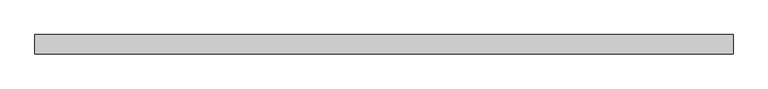
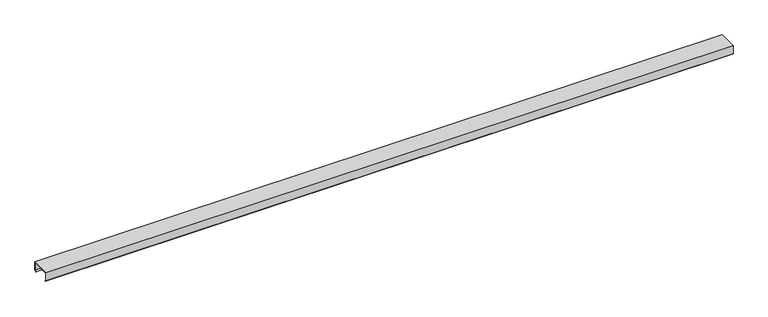
"""IFC4 building model written with IfcOpenShell, lengths in millimetres: proxy geometry, Generic Models 7:Generic Models 1:1:Generic Models 1:1 : Generic Models 7:Generic Models 1:337419:17 : Generic Models 7:Generic Models 1:1:Generic Models 1:1 : Generic Models 7:Generic Models 1:337419:306201."""

import ifcopenshell
import ifcopenshell.guid

model = None  # the IFC model being written
_history = None  # IfcOwnerHistory: only IFC2X3 demands one
_inside = {}  # id of a spatial element -> (the spatial element, [elements in it])
_under = {}  # id of a project, library or spatial element -> (it, [spatial elements below it])
_declared = {}  # id of a project -> (the project, [libraries it declares])
_typed = {}  # id of a type object -> (the type object, [elements of that type])
_made_of = {}  # id of a material, layer set ... -> (it, [elements and type objects made of it])


def new_model(schema):
    """Start an empty IFC model of exactly this schema.

    Asked for "IFC4X3", IfcOpenShell would pick the latest addendum, in which some entities
    have other attributes; the version numbers below select the first issue.
    IFC2X3 requires an IfcOwnerHistory on every rooted entity: one is made here for all.
    """
    global model, _history
    if schema == "IFC4X3":
        model = ifcopenshell.file(schema_version=(4, 3, 0, 0))
    else:
        model = ifcopenshell.file(schema=schema)
    _inside.clear()
    _under.clear()
    _declared.clear()
    _typed.clear()
    _made_of.clear()
    _history = None
    if model.schema == "IFC2X3":
        org = make("IfcOrganization", Name="unknown")
        user = make(
            "IfcPersonAndOrganization",
            ThePerson=make("IfcPerson", FamilyName="unknown"),
            TheOrganization=org,
        )
        app = make(
            "IfcApplication",
            ApplicationDeveloper=org,
            Version="unknown",
            ApplicationFullName="unknown",
            ApplicationIdentifier="unknown",
        )
        _history = make(
            "IfcOwnerHistory",
            OwningUser=user,
            OwningApplication=app,
            ChangeAction="ADDED",
            CreationDate=0,
        )
    return model


def make(cls, **values):
    """One entity of the class cls with the attributes given. An attribute that is None is left unset."""
    return model.create_entity(
        cls, **{name: value for name, value in values.items() if value is not None}
    )


def rooted(cls, **values):
    """An entity with a GlobalId (a new one), such as an element, a storey or a relation."""
    return make(cls, GlobalId=ifcopenshell.guid.new(), OwnerHistory=_history, **values)


def si_unit(unit_type, name, prefix=None):
    """IfcSIUnit, for example si_unit("LENGTHUNIT", "METRE", prefix="MILLI")."""
    return make("IfcSIUnit", UnitType=unit_type, Prefix=prefix, Name=name)


def assignment(units):
    """IfcUnitAssignment: the units of a project."""
    return None if units is None else make("IfcUnitAssignment", Units=units)


def point(xyz):
    """IfcCartesianPoint."""
    return None if xyz is None else make("IfcCartesianPoint", Coordinates=xyz)


def direction(xyz):
    """IfcDirection."""
    return None if xyz is None else make("IfcDirection", DirectionRatios=xyz)


def frame(location, z_axis=None, x_axis=None):
    """IfcAxis2Placement3D, a coordinate frame: its origin and axes. An axis left out is left unset."""
    return make(
        "IfcAxis2Placement3D",
        Location=point(location),
        Axis=direction(z_axis),
        RefDirection=direction(x_axis),
    )


def origin():
    """The frame at (0, 0, 0) with its axes left unset."""
    return frame((0.0, 0.0, 0.0))


def place(relative_to, where):
    """IfcLocalPlacement: puts the frame where relative to a parent placement (None: the world)."""
    return make(
        "IfcLocalPlacement", PlacementRelTo=relative_to, RelativePlacement=where
    )


def context(
    kind, dimensions, precision=None, world=None, true_north=None, identifier=None
):
    """IfcGeometricRepresentationContext, for example the 3D "Model" context."""
    return make(
        "IfcGeometricRepresentationContext",
        ContextIdentifier=identifier,
        ContextType=kind,
        CoordinateSpaceDimension=dimensions,
        Precision=precision,
        WorldCoordinateSystem=world,
        TrueNorth=true_north,
    )


def project(units=None, contexts=None):
    """IfcProject with its units and contexts."""
    return rooted(
        "IfcProject",
        Name="project",
        RepresentationContexts=contexts,
        UnitsInContext=assignment(units),
    )


def spatial(cls, under=None, at=None, **own):
    """A site, building, storey or space (cls), placed at a placement, below another one or the project."""
    s = rooted(cls, ObjectPlacement=at, **own)
    if under is not None:
        _under.setdefault(under.id(), (under, []))[1].append(s)
    return s


def polyline(points):
    """IfcPolyline through the points."""
    return make("IfcPolyline", Points=[point(p) for p in points])


def outline(outer, holes=None, kind="AREA"):
    """IfcArbitraryClosedProfileDef: a profile drawn as a closed curve; with holes, ...WithVoids."""
    if holes is None:
        return make("IfcArbitraryClosedProfileDef", ProfileType=kind, OuterCurve=outer)
    return make(
        "IfcArbitraryProfileDefWithVoids",
        ProfileType=kind,
        OuterCurve=outer,
        InnerCurves=holes,
    )


def extrude(swept, where, along, depth):
    """IfcExtrudedAreaSolid: the profile swept, set in the frame where, extruded along a direction by depth."""
    return make(
        "IfcExtrudedAreaSolid",
        SweptArea=swept,
        Position=where,
        ExtrudedDirection=direction(along),
        Depth=depth,
    )


def shape(context_of_items, identifier, shape_type, items):
    """IfcShapeRepresentation: the items that make up one representation, for example the "Body"."""
    return make(
        "IfcShapeRepresentation",
        ContextOfItems=context_of_items,
        RepresentationIdentifier=identifier,
        RepresentationType=shape_type,
        Items=items,
    )


def source(mapping_origin, context_of_items, identifier, shape_type, items):
    """IfcRepresentationMap: a shape defined once, which mapped items show again and again."""
    return make(
        "IfcRepresentationMap",
        MappingOrigin=mapping_origin,
        MappedRepresentation=shape(context_of_items, identifier, shape_type, items),
    )


def transform(
    local_origin,
    x_axis=None,
    y_axis=None,
    z_axis=None,
    scale=None,
    scale2=None,
    scale3=None,
    uniform=True,
):
    """IfcCartesianTransformationOperator3D, or its non-uniform kind. x_axis, y_axis, z_axis: its Axis1, 2, 3."""
    if uniform:
        return make(
            "IfcCartesianTransformationOperator3D",
            Axis1=direction(x_axis),
            Axis2=direction(y_axis),
            LocalOrigin=point(local_origin),
            Scale=scale,
            Axis3=direction(z_axis),
        )
    return make(
        "IfcCartesianTransformationOperator3DnonUniform",
        Axis1=direction(x_axis),
        Axis2=direction(y_axis),
        LocalOrigin=point(local_origin),
        Scale=scale,
        Axis3=direction(z_axis),
        Scale2=scale2,
        Scale3=scale3,
    )


def mapped(mapping_source, mapping_target):
    """IfcMappedItem: shows the shape of a source again, moved by a transform."""
    return make(
        "IfcMappedItem", MappingSource=mapping_source, MappingTarget=mapping_target
    )


def made_of(thing, what):
    """Note that an element or type object is made of a material, layer set ...; save() writes the relation."""
    if what is not None:
        _made_of.setdefault(what.id(), (what, []))[1].append(thing)
    return thing


def element(
    cls,
    number,
    at=None,
    inside=None,
    cuts=None,
    type_object=None,
    material=None,
    context=None,
    identifier="Body",
    shape_type=None,
    held_by="IfcProductDefinitionShape",
    body=None,
    shapes=None,
    **own,
):
    """One element of the class cls, such as IfcWall. Its Tag is "e" and its number.

    at: its placement. inside: the storey or other place that contains it. cuts: it is an
    opening in that element (IfcRelVoidsElement). A single representation is given by context,
    identifier, shape_type and body (its items); several are given by shapes. held_by: the class
    of the entity that holds the representations. save() writes the other relations.
    """
    e = rooted(cls, Tag="e%d" % number, ObjectPlacement=at, **own)
    if body is not None:
        shapes = [shape(context, identifier, shape_type, body)]
    if shapes is not None:
        e.Representation = make(held_by, Representations=shapes)
    if inside is not None:
        _inside.setdefault(inside.id(), (inside, []))[1].append(e)
    if cuts is not None:
        rooted(
            "IfcRelVoidsElement", RelatingBuildingElement=cuts, RelatedOpeningElement=e
        )
    if type_object is not None:
        _typed.setdefault(type_object.id(), (type_object, []))[1].append(e)
    return made_of(e, material)


def aggregate(whole, parts):
    """IfcRelAggregates: a whole, such as a stair, and the parts it consists of."""
    return rooted("IfcRelAggregates", RelatingObject=whole, RelatedObjects=parts)


def save(model, path):
    """Write the relations noted so far, then the file.

    IfcRelAggregates (storeys below a building ...), IfcRelContainedInSpatialStructure (elements
    in a storey), IfcRelDefinesByType, IfcRelAssociatesMaterial and IfcRelDeclares: one each for
    every whole, place, type object, material and project.
    """
    for whole, parts in _under.values():
        aggregate(whole, parts)
    for where, things in _inside.values():
        rooted(
            "IfcRelContainedInSpatialStructure",
            RelatedElements=things,
            RelatingStructure=where,
        )
    for kind, things in _typed.values():
        rooted("IfcRelDefinesByType", RelatedObjects=things, RelatingType=kind)
    for what, things in _made_of.values():
        rooted("IfcRelAssociatesMaterial", RelatedObjects=things, RelatingMaterial=what)
    for by, libraries in _declared.values():
        rooted("IfcRelDeclares", RelatingContext=by, RelatedDefinitions=libraries)
    model.write(path)


def generic_models_0e7b4f9b(model_context):
    return source(origin(), model_context, "Body", "SweptSolid", [
        extrude(outline(polyline([(-578797.4913841, 6128.940625), (-578797.4913841, 6040.040625), (-578812.0845307, 6027.7955211), (-578813.870275, 6029.9236883), (-578800.2695091, 6041.336086), (-578800.2695091, 6126.1625), (-578997.9132591, 6126.1625), (-578997.9132591, 6041.336086), (-578984.3124931, 6029.9236883), (-578986.0982374, 6027.7955211), (-579000.6913841, 6040.040625), (-579000.6913841, 6128.940625), (-578797.4913841, 6128.940625)])), frame((574430.911724, 0.0, 0.0), z_axis=(1.0, 0.0, 0.0), x_axis=(0.0, 1.0, 0.0)), (0.0, 0.0, 1.0), 7315.2),
    ])


if __name__ == "__main__":
    model = new_model("IFC4")
    model_context = context("Model", 3, world=origin())
    ifc_project = project(units=[si_unit("LENGTHUNIT", "METRE", prefix="MILLI")], contexts=[model_context])
    site = spatial("IfcSite", under=ifc_project)
    building = spatial("IfcBuilding", under=site)
    placement = place(None, origin())
    generic_models_shape = generic_models_0e7b4f9b(model_context)
    element("IfcBuildingElementProxy", 1, Name="Generic Models 7:Generic Models 1:1:Generic Models 1:1 : Generic Models 7:Generic Models 1:337419:17 : Generic Models 7:Generic Models 1:1:Generic Models 1:1 : Generic Models 7:Generic Models 1:337419:306201", ObjectType="Generic Models 7:Generic Models 1:1:Generic Models 1:1 : Generic Models 7:Generic Models 1:337419:17 : Generic Models 7:Generic Models 1:1:Generic Models 1:1 : Generic Models 7:Generic Models 1:337419:306201", at=placement, inside=building, context=model_context, shape_type="MappedRepresentation", body=[
        mapped(generic_models_shape, transform((0.0, 0.0, 0.0), x_axis=(1.0, 0.0, 0.0), y_axis=(0.0, 1.0, 0.0), z_axis=(0.0, 0.0, 1.0))),
    ])
    save(model, "model.ifc")

# Revit data of these elements
# Type "Generic Models 7:Generic Models 1:1:Generic Models 1:1 : Generic Models 7:Generic Models 1:337419:17 : Generic Models 7:Generic Models 1:1:Generic Models 1:1 : Generic Models 7:Generic Models 1:337419:306201"
#   NameOverride = "Generic Models 7:Generic Models 1:1:Generic Models 1:1 : Generic Models 7:Generic Models 1:337419:306201"
#   ObjectTypeOverride = "Generic Models 1:1 : Generic Models 7:Generic Models 1:337419"
#   Reference = "Generic Models 1"
#   Tag = "306201"
# Element 1 (IfcBuildingElementProxy, "Generic Models 7:Generic Models 1:1:Generic Models 1:1 : Generic Models 7:Generic Models 1:337419:17 : Generic Models 7:Generic Models 1:1:Generic Models 1:1 : Generic Models 7:Generic Models 1:337419:306201")
#   Materials on its faces: "'ZEE' SECTION (8.0x3.5Z - SEE STRUCT. DWGS)"
# Materials
#   "'ZEE' SECTION (8.0x3.5Z - SEE STRUCT. DWGS)": class "Unassigned", colour RGB 210 209 208, transparency 0, Keynote = "M05121300.02", Cost = 0
